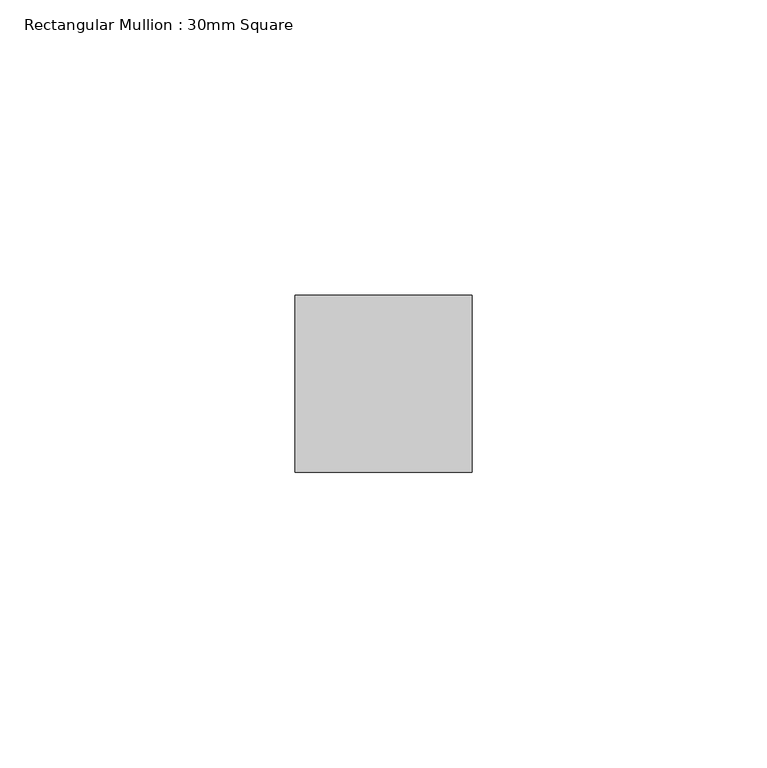
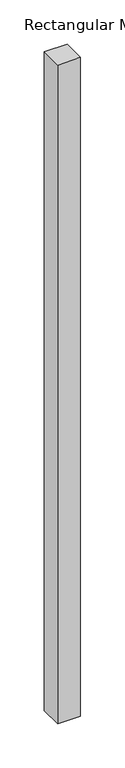
"""IFC4 building model written with IfcOpenShell, lengths in millimetres: member geometry, Rectangular Mullion : 30mm Square."""

from ifc_helpers import new_model, si_unit, frame, origin, place, context, project, spatial, polyline, outline, extrude, source, transform, mapped, element, save


def rectangular_mullion_30mm_square_29e3a418(model_context):
    return source(origin(), model_context, "Body", "SweptSolid", [
        extrude(outline(polyline([(15.0, 15.0), (15.0, -15.0), (-15.0, -15.0), (-15.0, 15.0), (15.0, 15.0)])), frame((0.0, 0.0, -908.9542032), z_axis=(0.0, 0.0, 1.0), x_axis=(1.0, 0.0, 0.0)), (0.0, 0.0, 1.0), 908.9542032),
    ])


if __name__ == "__main__":
    model = new_model("IFC4")
    model_context = context("Model", 3, world=origin())
    ifc_project = project(units=[si_unit("LENGTHUNIT", "METRE", prefix="MILLI")], contexts=[model_context])
    site = spatial("IfcSite", under=ifc_project)
    building = spatial("IfcBuilding", under=site)
    placement = place(None, origin())
    rectangular_mullion_30mm_square_shape = rectangular_mullion_30mm_square_29e3a418(model_context)
    element("IfcMember", 1, ObjectType="Rectangular Mullion : 30mm Square", at=placement, inside=building, context=model_context, shape_type="MappedRepresentation", body=[
        mapped(rectangular_mullion_30mm_square_shape, transform((0.0, 0.0, 0.0), x_axis=(1.0, 0.0, 0.0), y_axis=(0.0, 1.0, 0.0), z_axis=(0.0, 0.0, 1.0))),
    ])
    save(model, "model.ifc")

# Revit data of these elements
# Type "Rectangular Mullion : 30mm Square"
#   built-in parameter 1007304 = 0.0984252 (stored number, unit not read)
#   built-in parameter 1007301 = 0.0492126 (stored number, unit not read)
#   built-in parameter 1007300 = 0.0492126 (stored number, unit not read)
# Element 1 (IfcMember, "Rectangular Mullion : 30mm Square")
#   Materials on its faces: "Aluminum"
# Materials
#   "Aluminum": class "Metal", colour RGB 244 244 244, transparency 0, Description = "Aluminum 6061", Cost = 0
